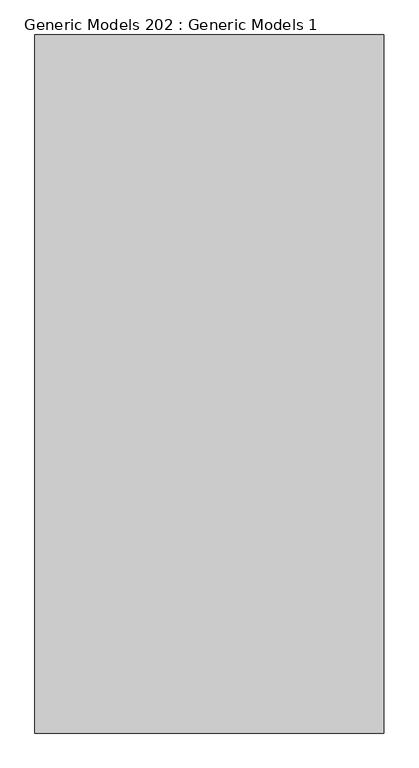
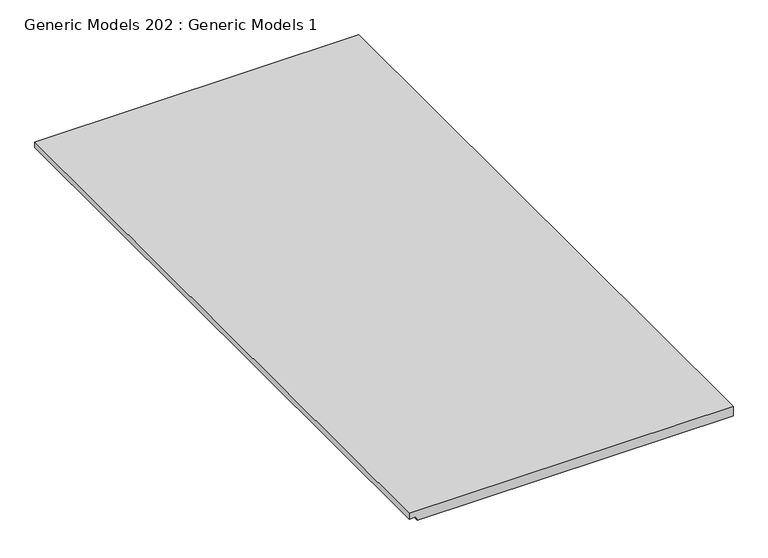
"""IFC4 building model written with IfcOpenShell, lengths in millimetres: proxy geometry, Generic Models 202 : Generic Models 1."""

import ifcopenshell
import ifcopenshell.guid

model = None  # the IFC model being written
_history = None  # IfcOwnerHistory: only IFC2X3 demands one
_inside = {}  # id of a spatial element -> (the spatial element, [elements in it])
_under = {}  # id of a project, library or spatial element -> (it, [spatial elements below it])
_declared = {}  # id of a project -> (the project, [libraries it declares])
_typed = {}  # id of a type object -> (the type object, [elements of that type])
_made_of = {}  # id of a material, layer set ... -> (it, [elements and type objects made of it])


def new_model(schema):
    """Start an empty IFC model of exactly this schema.

    Asked for "IFC4X3", IfcOpenShell would pick the latest addendum, in which some entities
    have other attributes; the version numbers below select the first issue.
    IFC2X3 requires an IfcOwnerHistory on every rooted entity: one is made here for all.
    """
    global model, _history
    if schema == "IFC4X3":
        model = ifcopenshell.file(schema_version=(4, 3, 0, 0))
    else:
        model = ifcopenshell.file(schema=schema)
    _inside.clear()
    _under.clear()
    _declared.clear()
    _typed.clear()
    _made_of.clear()
    _history = None
    if model.schema == "IFC2X3":
        org = make("IfcOrganization", Name="unknown")
        user = make(
            "IfcPersonAndOrganization",
            ThePerson=make("IfcPerson", FamilyName="unknown"),
            TheOrganization=org,
        )
        app = make(
            "IfcApplication",
            ApplicationDeveloper=org,
            Version="unknown",
            ApplicationFullName="unknown",
            ApplicationIdentifier="unknown",
        )
        _history = make(
            "IfcOwnerHistory",
            OwningUser=user,
            OwningApplication=app,
            ChangeAction="ADDED",
            CreationDate=0,
        )
    return model


def make(cls, **values):
    """One entity of the class cls with the attributes given. An attribute that is None is left unset."""
    return model.create_entity(
        cls, **{name: value for name, value in values.items() if value is not None}
    )


def rooted(cls, **values):
    """An entity with a GlobalId (a new one), such as an element, a storey or a relation."""
    return make(cls, GlobalId=ifcopenshell.guid.new(), OwnerHistory=_history, **values)


def si_unit(unit_type, name, prefix=None):
    """IfcSIUnit, for example si_unit("LENGTHUNIT", "METRE", prefix="MILLI")."""
    return make("IfcSIUnit", UnitType=unit_type, Prefix=prefix, Name=name)


def assignment(units):
    """IfcUnitAssignment: the units of a project."""
    return None if units is None else make("IfcUnitAssignment", Units=units)


def point(xyz):
    """IfcCartesianPoint."""
    return None if xyz is None else make("IfcCartesianPoint", Coordinates=xyz)


def direction(xyz):
    """IfcDirection."""
    return None if xyz is None else make("IfcDirection", DirectionRatios=xyz)


def frame(location, z_axis=None, x_axis=None):
    """IfcAxis2Placement3D, a coordinate frame: its origin and axes. An axis left out is left unset."""
    return make(
        "IfcAxis2Placement3D",
        Location=point(location),
        Axis=direction(z_axis),
        RefDirection=direction(x_axis),
    )


def origin():
    """The frame at (0, 0, 0) with its axes left unset."""
    return frame((0.0, 0.0, 0.0))


def place(relative_to, where):
    """IfcLocalPlacement: puts the frame where relative to a parent placement (None: the world)."""
    return make(
        "IfcLocalPlacement", PlacementRelTo=relative_to, RelativePlacement=where
    )


def context(
    kind, dimensions, precision=None, world=None, true_north=None, identifier=None
):
    """IfcGeometricRepresentationContext, for example the 3D "Model" context."""
    return make(
        "IfcGeometricRepresentationContext",
        ContextIdentifier=identifier,
        ContextType=kind,
        CoordinateSpaceDimension=dimensions,
        Precision=precision,
        WorldCoordinateSystem=world,
        TrueNorth=true_north,
    )


def project(units=None, contexts=None):
    """IfcProject with its units and contexts."""
    return rooted(
        "IfcProject",
        Name="project",
        RepresentationContexts=contexts,
        UnitsInContext=assignment(units),
    )


def spatial(cls, under=None, at=None, **own):
    """A site, building, storey or space (cls), placed at a placement, below another one or the project."""
    s = rooted(cls, ObjectPlacement=at, **own)
    if under is not None:
        _under.setdefault(under.id(), (under, []))[1].append(s)
    return s


def polyline(points):
    """IfcPolyline through the points."""
    return make("IfcPolyline", Points=[point(p) for p in points])


def outline(outer, holes=None, kind="AREA"):
    """IfcArbitraryClosedProfileDef: a profile drawn as a closed curve; with holes, ...WithVoids."""
    if holes is None:
        return make("IfcArbitraryClosedProfileDef", ProfileType=kind, OuterCurve=outer)
    return make(
        "IfcArbitraryProfileDefWithVoids",
        ProfileType=kind,
        OuterCurve=outer,
        InnerCurves=holes,
    )


def extrude(swept, where, along, depth):
    """IfcExtrudedAreaSolid: the profile swept, set in the frame where, extruded along a direction by depth."""
    return make(
        "IfcExtrudedAreaSolid",
        SweptArea=swept,
        Position=where,
        ExtrudedDirection=direction(along),
        Depth=depth,
    )


def shape(context_of_items, identifier, shape_type, items):
    """IfcShapeRepresentation: the items that make up one representation, for example the "Body"."""
    return make(
        "IfcShapeRepresentation",
        ContextOfItems=context_of_items,
        RepresentationIdentifier=identifier,
        RepresentationType=shape_type,
        Items=items,
    )


def source(mapping_origin, context_of_items, identifier, shape_type, items):
    """IfcRepresentationMap: a shape defined once, which mapped items show again and again."""
    return make(
        "IfcRepresentationMap",
        MappingOrigin=mapping_origin,
        MappedRepresentation=shape(context_of_items, identifier, shape_type, items),
    )


def transform(
    local_origin,
    x_axis=None,
    y_axis=None,
    z_axis=None,
    scale=None,
    scale2=None,
    scale3=None,
    uniform=True,
):
    """IfcCartesianTransformationOperator3D, or its non-uniform kind. x_axis, y_axis, z_axis: its Axis1, 2, 3."""
    if uniform:
        return make(
            "IfcCartesianTransformationOperator3D",
            Axis1=direction(x_axis),
            Axis2=direction(y_axis),
            LocalOrigin=point(local_origin),
            Scale=scale,
            Axis3=direction(z_axis),
        )
    return make(
        "IfcCartesianTransformationOperator3DnonUniform",
        Axis1=direction(x_axis),
        Axis2=direction(y_axis),
        LocalOrigin=point(local_origin),
        Scale=scale,
        Axis3=direction(z_axis),
        Scale2=scale2,
        Scale3=scale3,
    )


def mapped(mapping_source, mapping_target):
    """IfcMappedItem: shows the shape of a source again, moved by a transform."""
    return make(
        "IfcMappedItem", MappingSource=mapping_source, MappingTarget=mapping_target
    )


def made_of(thing, what):
    """Note that an element or type object is made of a material, layer set ...; save() writes the relation."""
    if what is not None:
        _made_of.setdefault(what.id(), (what, []))[1].append(thing)
    return thing


def element(
    cls,
    number,
    at=None,
    inside=None,
    cuts=None,
    type_object=None,
    material=None,
    context=None,
    identifier="Body",
    shape_type=None,
    held_by="IfcProductDefinitionShape",
    body=None,
    shapes=None,
    **own,
):
    """One element of the class cls, such as IfcWall. Its Tag is "e" and its number.

    at: its placement. inside: the storey or other place that contains it. cuts: it is an
    opening in that element (IfcRelVoidsElement). A single representation is given by context,
    identifier, shape_type and body (its items); several are given by shapes. held_by: the class
    of the entity that holds the representations. save() writes the other relations.
    """
    e = rooted(cls, Tag="e%d" % number, ObjectPlacement=at, **own)
    if body is not None:
        shapes = [shape(context, identifier, shape_type, body)]
    if shapes is not None:
        e.Representation = make(held_by, Representations=shapes)
    if inside is not None:
        _inside.setdefault(inside.id(), (inside, []))[1].append(e)
    if cuts is not None:
        rooted(
            "IfcRelVoidsElement", RelatingBuildingElement=cuts, RelatedOpeningElement=e
        )
    if type_object is not None:
        _typed.setdefault(type_object.id(), (type_object, []))[1].append(e)
    return made_of(e, material)


def aggregate(whole, parts):
    """IfcRelAggregates: a whole, such as a stair, and the parts it consists of."""
    return rooted("IfcRelAggregates", RelatingObject=whole, RelatedObjects=parts)


def save(model, path):
    """Write the relations noted so far, then the file.

    IfcRelAggregates (storeys below a building ...), IfcRelContainedInSpatialStructure (elements
    in a storey), IfcRelDefinesByType, IfcRelAssociatesMaterial and IfcRelDeclares: one each for
    every whole, place, type object, material and project.
    """
    for whole, parts in _under.values():
        aggregate(whole, parts)
    for where, things in _inside.values():
        rooted(
            "IfcRelContainedInSpatialStructure",
            RelatedElements=things,
            RelatingStructure=where,
        )
    for kind, things in _typed.values():
        rooted("IfcRelDefinesByType", RelatedObjects=things, RelatingType=kind)
    for what, things in _made_of.values():
        rooted("IfcRelAssociatesMaterial", RelatedObjects=things, RelatingMaterial=what)
    for by, libraries in _declared.values():
        rooted("IfcRelDeclares", RelatingContext=by, RelatedDefinitions=libraries)
    model.write(path)


def generic_models_202_generic_models_1_9e5f3db3(model_context):
    return source(origin(), model_context, "Body", "SweptSolid", [
        extrude(outline(polyline([(328.8831074, 52679.7897516), (317.7706074, 52679.7897516), (317.7706074, 52692.4897516), (309.8331074, 52695.3787653), (309.8331074, 53289.3897516), (328.8831074, 53289.3897516), (328.8831074, 52679.7897516)])), frame((0.0, 0.0, 0.0), z_axis=(0.0, 1.0, 0.0), x_axis=(0.0, 0.0, 1.0)), (0.0, 0.0, 1.0), 1219.2),
    ])


if __name__ == "__main__":
    model = new_model("IFC4")
    model_context = context("Model", 3, world=origin())
    ifc_project = project(units=[si_unit("LENGTHUNIT", "METRE", prefix="MILLI")], contexts=[model_context])
    site = spatial("IfcSite", under=ifc_project)
    building = spatial("IfcBuilding", under=site)
    placement = place(None, origin())
    generic_models_202_generic_models_1_shape = generic_models_202_generic_models_1_9e5f3db3(model_context)
    element("IfcBuildingElementProxy", 1, Name="Generic Models 202 : Generic Models 1", ObjectType="Generic Models 202 : Generic Models 1", at=placement, inside=building, context=model_context, shape_type="MappedRepresentation", body=[
        mapped(generic_models_202_generic_models_1_shape, transform((0.0, 0.0, 0.0), x_axis=(1.0, 0.0, 0.0), y_axis=(0.0, 1.0, 0.0), z_axis=(0.0, 0.0, 1.0))),
    ])
    save(model, "model.ifc")

# Revit data of these elements
# Element 1 (IfcBuildingElementProxy, "Generic Models 202 : Generic Models 1")
#   Materials on its faces: "EXISTING ACT CEILING"
# Materials
#   "EXISTING ACT CEILING": class "Generic", colour RGB 255 255 255, transparency 0, Cost = 0
